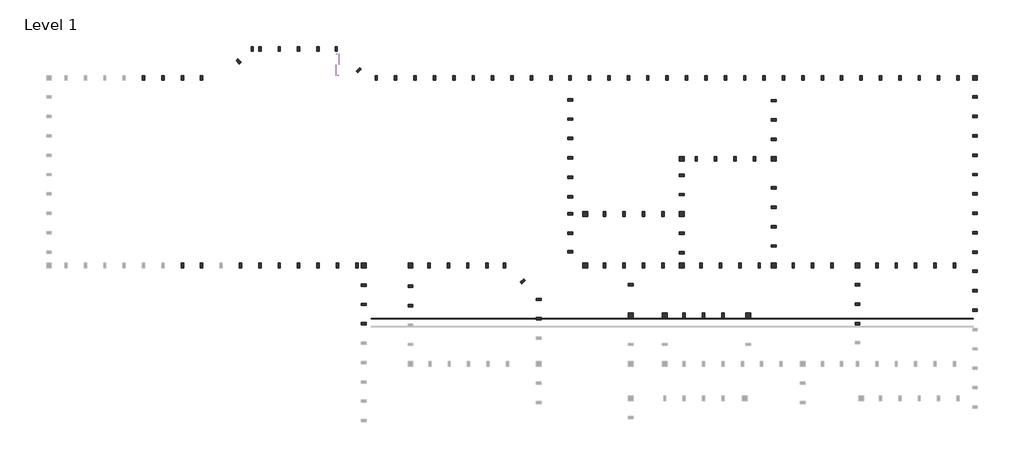
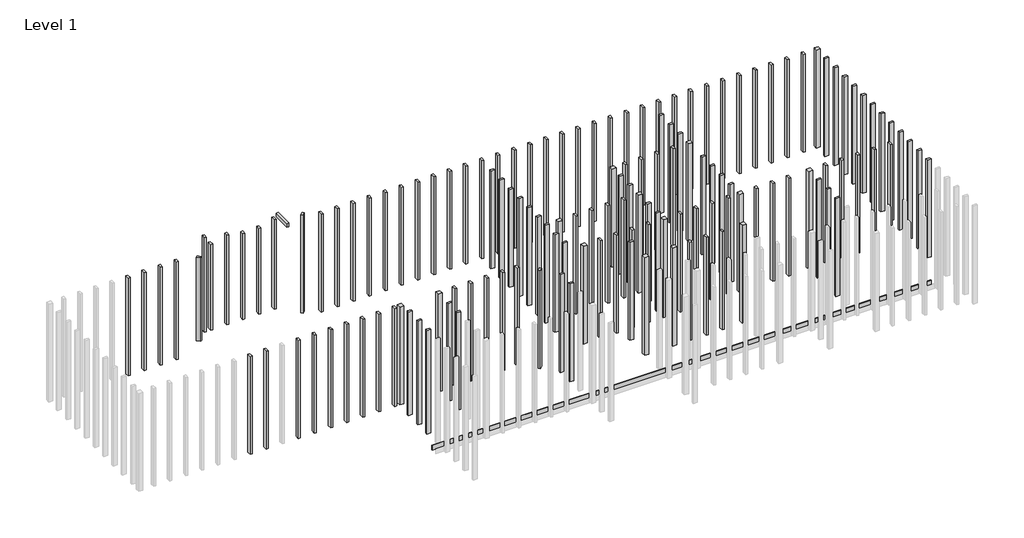
# One storey, part 2 of 2: 142 columns, 3 beams.
# Revit data of these elements (continued)
# Elements 4, 5, 6, 7, 8, 9, 10, 11, 12, 13, 14, 15, 16, 17, 18, 19, 20, 21, 22, 23, 24, 25, 26, 27, 28, 29, 30, 31, 32, 33, 34, 35, 36, 37, 38, 39, 40, 41, 42, 43, 44, 45, 46, 47, 48, 49, 50, 51, 52, 53, 54, 55, 56, 57, 58, 59, 60, 61, 62, 63, 64, 65, 66, 67, 68, 69, 70, 71, 72, 73, 74, 75, 76, 77, 78, 79, 80, 81, 82, 83, 84, 85, 86, 87, 88, 89, 90, 91, 92, 93, 94, 95, 96, 97, 98, 99, 100, 101, 102, 103, 104, 105, 106, 107, 108, 109, 110, 111, 112, 113, 114, 129, 130, 131, 132, 133, 134, 135, 136, 137, 138, 139, 140, 141, 142, 143, 144, 145 (IfcColumn, "Timber-Column : BLDG 6241 Wall Struds 2\"x4\"")
#   Comments = ""
#   Structural Material = Softwood, Lumber
#   Phase Created = New Construction
#   Materials on its faces: "Softwood, Lumber"
# Elements 115, 116, 117, 118, 119, 120, 121, 122, 123, 124, 125, 126, 127, 128 (IfcColumn, "Timber-Column : BLDG 6241 Wall Struds 4\"x4\"")
#   Comments = ""
#   Structural Material = Softwood, Lumber
#   Phase Created = New Construction
#   Materials on its faces: "Softwood, Lumber"
# Materials
#   "Softwood, Lumber": class "Wood", colour RGB 223 192 134, transparency 0, Description = "Pinus Echinata", Cost = 0
#   "Plywood, Sheathing": class "Wood", colour RGB 212 179 113, transparency 0, Description = "Plywood, sheathing grade", Cost = 0
